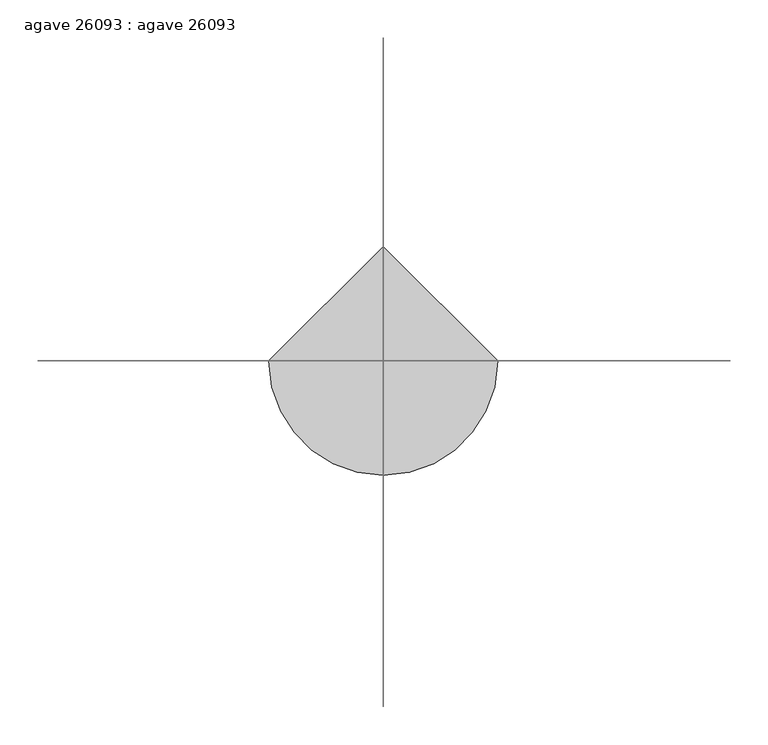
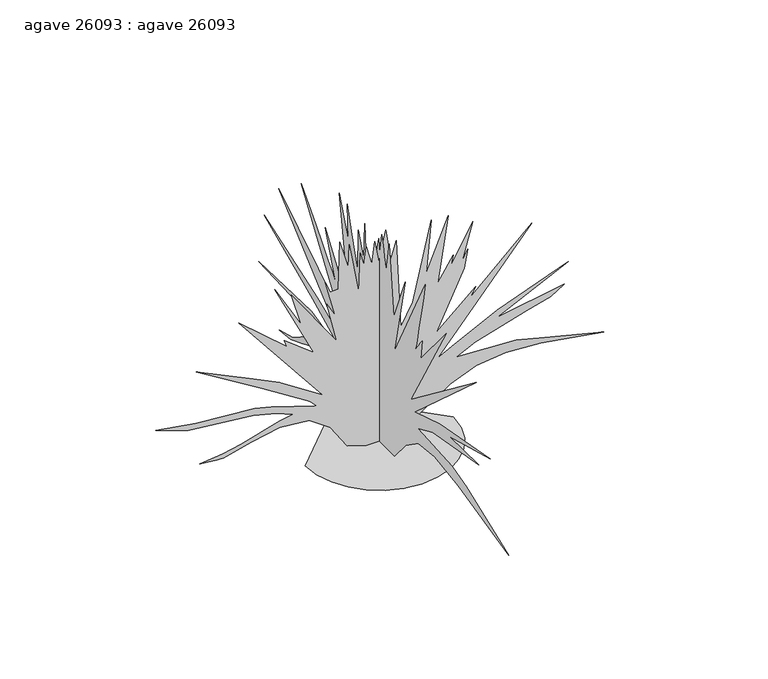
"""IFC4 building model written with IfcOpenShell, lengths in millimetres: proxy geometry, agave 26093 : agave 26093."""

from ifc_helpers import new_model, si_unit, origin, place, context, project, spatial, triangles, source, transform, mapped, element, save


def agave_26093_agave_26093_93a2a214(model_context):
    return source(origin(), model_context, "Body", "Tessellation", [
        triangles([(-150.7087333, 0.0, 9.4e-06), (-146.7244834, -34.5323444, 9.4e-06), (-135.3772836, -66.2450299, 9.4e-06), (-117.5759356, -94.2289958, 9.4e-06), (-94.2289958, -117.5759356, 9.4e-06), (-66.2450299, -135.3772836, 9.4e-06), (-34.5323444, -146.7244834, 9.4e-06), (6.6e-06, -150.7087333, 9.4e-06), (34.5323444, -146.7244834, 9.4e-06), (66.2450299, -135.3772836, 9.4e-06), (94.2289958, -117.5759356, 9.4e-06), (117.5759356, -94.2289958, 9.4e-06), (135.3772836, -66.2450299, 9.4e-06), (146.7244834, -34.5323444, 9.4e-06), (150.7087333, 1.32e-05, 9.4e-06), (-1.98e-05, 150.7087333, 9.4e-06), (-24.9398476, 1.1e-06, 2.5e-06), (-65.4258802, 2.1e-06, 13.141818), (-99.6620581, 5e-07, 65.0964399), (-143.0435126, 6e-07, 95.6658721), (-202.3246234, 2.8e-06, 101.1403381), (-259.7355268, 6e-06, 89.1792132), (-316.7763402, 9.4e-06, 74.9889865), (-329.6211594, 9.9e-06, 75.5035945), (-365.3285002, 1.12e-05, 79.1975187), (-318.313056, 8.9e-06, 84.1103911), (-282.3389982, 6.9e-06, 91.7898278), (-203.1008479, 2e-06, 114.8573697), (-175.7107319, 5e-07, 119.829677), (-208.3624635, 1.2e-06, 133.0887423), (-256.7688111, 2.5e-06, 145.787731), (-389.2832517, 7.5e-06, 160.0767662), (-455.2115313, 9e-06, 182.6248811), (-373.9467241, 6.3e-06, 169.0808314), (-253.2813787, 1.6e-06, 159.2306877), (-220.3573709, 6e-07, 151.0805947), (-127.6907252, -1.6e-06, 121.0610699), (-140.4735387, -1.9e-06, 135.3043865), (-238.3492232, -1.3e-06, 197.06021), (-372.7148226, -4e-07, 279.8955245), (-256.342093, -2.1e-06, 224.048243), (-204.0302424, -2.9e-06, 198.6317166), (-115.3780683, -3.3e-06, 140.7615752), (-286.5249345, -8.6e-06, 355.0033673), (-188.0233888, -7.9e-06, 270.045399), (-192.9487059, -8.5e-06, 284.8205873), (-133.8471808, -8.3e-06, 238.0324729), (-212.6492294, -1.47e-05, 401.7927715), (-158.472758, -1.14e-05, 306.9846414), (-179.4046562, -1.47e-05, 378.3993593), (-87.0585669, -1.09e-05, 246.6514781), (-106.7590813, -1.52e-05, 332.8418567), (-89.5210982, -1.41e-05, 302.0595786), (-110.4530055, -1.79e-05, 380.860619), (-99.717687, -1.69e-05, 356.9287222), (-83.2732056, -1.76e-05, 356.9490335), (-80.9021112, -2.37e-05, 457.2003633), (-63.426897, -2.09e-05, 396.9718449), (-61.2016014, -2.38e-05, 444.8864347), (-41.5013458, -1.82e-05, 335.3031163), (-39.0385601, -2.33e-05, 419.0317629), (-31.650966, -2.19e-05, 390.7107445), (-26.7259009, -2.44e-05, 428.8818884), (-15.6443803, -2.24e-05, 387.0175833), (-9.4879996, -2.54e-05, 433.8069511), (-0.8690236, -2.3e-05, 387.0175833), (12.6750416, -2.74e-05, 451.043399), (23.7565623, -2.39e-05, 383.3244221), (34.8381601, -2.66e-05, 420.261121), (43.4571494, -1.56e-05, 230.6448788), (68.0824677, -1.94e-05, 276.2023633), (105.4982208, -3.08e-05, 439.9537416), (95.1708261, -2.38e-05, 329.146152), (140.4829403, -3.22e-05, 436.9539974), (118.5650104, -2.3e-05, 299.5957755), (150.578436, -2.74e-05, 348.8489465), (145.6533642, -2.58e-05, 326.6848924), (189.9794467, -3.25e-05, 406.7178343), (167.81641, -2.69e-05, 327.9167939), (180.1290669, -2.88e-05, 351.3102061), (173.4681726, -2.62e-05, 313.009528), (116.102479, -1.66e-05, 193.7063995), (196.1359024, -2.44e-05, 265.1203362), (183.8229911, -2.26e-05, 244.1889286), (310.6447741, -3.51e-05, 361.1603316), (118.5650104, -1.34e-05, 138.2987895), (158.4747927, -1.63e-05, 158.0775423), (240.4617396, -2.24e-05, 198.6317166), (384.5207517, -3.19e-05, 252.8079337), (239.2306011, -2.13e-05, 182.6248811), (376.7864491, -2.88e-05, 206.3655105), (349.174072, -2.66e-05, 189.8819236), (300.4111145, -2.36e-05, 176.0696308), (195.4584909, -1.73e-05, 146.0828801), (156.7348917, -1.44e-05, 127.2172711), (278.6305944, -1.94e-05, 121.0610699), (336.3953462, -2.1e-05, 106.1004551), (457.1673348, -2.45e-05, 75.5035945), (329.0750444, -2.01e-05, 96.2046111), (257.431743, -1.73e-05, 101.1027496), (197.4574787, -1.42e-05, 94.105802), (144.7537007, -1.07e-05, 73.3684686), (86.5066293, -5.8e-06, 34.1325482), (33.0588878, -1.4e-06, 0.0), (9e-07, 20.0836192, 9.1e-06), (2.1e-06, 47.8000438, 9.9e-06), (3.7e-06, 68.4088604, 20.0829062), (6.2e-06, 99.6950775, 59.1195655), (8.3e-06, 132.7178983, 80.7177112), (1.03e-05, 174.2748821, 84.8467378), (1.15e-05, 208.5839434, 72.8693576), (1.35e-05, 272.2425033, 45.8366235), (1.48e-05, 311.9833551, 30.2844433), (1.65e-05, 353.3269798, 25.0212039), (1.48e-05, 305.3793614, 38.860505), (1.34e-05, 249.7515432, 74.8251566), (1.18e-05, 199.8564965, 97.660536), (1.01e-05, 161.2479701, 96.4354927), (1.17e-05, 188.527337, 110.366392), (1.51e-05, 256.1160167, 122.0234748), (2.29e-05, 425.717038, 129.5510222), (1.47e-05, 238.8183625, 134.6051196), (1.09e-05, 164.9452008, 118.743824), (8.2e-06, 119.3844099, 96.4354927), (1.1e-05, 159.9457058, 127.6671074), (1.54e-05, 233.8196305, 165.2718342), (2.53e-05, 406.273312, 240.4952587), (1.5e-05, 217.8867004, 177.6998184), (1.1e-05, 147.7036569, 148.1491784), (2.57e-05, 354.5588814, 329.146152), (1.25e-05, 146.2032761, 198.5547591), (2.38e-05, 274.5259576, 388.2494848), (2.18e-05, 248.7817623, 359.4966614), (1.99e-05, 223.9913424, 331.6328098), (1.81e-05, 201.1074557, 305.5495545), (1.65e-05, 181.0833509, 282.1358129), (1.52e-05, 164.872549, 262.2780679), (1.42e-05, 153.4283166, 246.8711776), (1.37e-05, 147.7036569, 236.8013344), (1.88e-05, 190.798601, 345.1532418), (1.51e-05, 148.9134577, 283.7461616), (1.48e-05, 144.9251474, 278.3410409), (1.44e-05, 140.1001603, 272.7403471), (1.4e-05, 134.5776867, 266.9770725), (1.35e-05, 128.4971803, 261.086807), (1.31e-05, 121.9980766, 255.0974924), (1.26e-05, 115.2200837, 249.0439011), (1.21e-05, 108.3028915, 242.95779), (1.97e-05, 140.3160628, 449.8114975), (1.58e-05, 109.53403, 367.3172959), (1.82e-05, 113.2279542, 442.4251751), (1.61e-05, 98.452766, 393.1745476), (1.29e-05, 75.0583319, 320.5279281), (1.55e-05, 73.826939, 410.4109955), (1.32e-05, 55.357822, 358.699072), (1.53e-05, 51.6638932, 437.5001123), (1.36e-05, 47.2595336, 384.1829453), (1.1e-05, 27.0383205, 327.9167939), (1.31e-05, 1.1814591, 436.2682108), (1.2e-05, -1.2811313, 405.4859327), (1.3e-05, -8.5500533, 450.4566616), (1.25e-05, -11.9783704, 436.1437634), (1.19e-05, -15.2441015, 422.2677209), (1.14e-05, -18.1847128, 409.2629188), (1.09e-05, -20.6375916, 397.5687561), (1.05e-05, -22.4401819, 387.6195451), (1.03e-05, -23.4298925, 379.852214), (1.01e-05, -23.4441676, 374.7036547), (1.18e-05, -34.5257405, 446.1183363), (6.6e-06, -50.5323262, 298.3664174), (7.8e-06, -92.3958773, 399.3315119), (4.4e-06, -52.9948575, 225.7198161), (5.7e-06, -162.5786665, 436.2682108), (5.1e-06, -155.9520543, 404.0000133), (4.4e-06, -149.5159464, 372.9078704), (3.8e-06, -143.4613468, 344.1651844), (3.3e-06, -137.9787509, 318.9480463), (2.9e-06, -133.2591716, 298.4324563), (2.7e-06, -129.4933677, 283.7918891), (2.6e-06, -126.87158, 276.2023633), (2.5e-06, -126.0089964, 274.2135312), (2.5e-06, -127.1682462, 275.2524031), (2.5e-06, -130.0120315, 278.8160301), (2.5e-06, -134.204054, 284.398956), (2.5e-06, -139.4067433, 291.4957067), (2.4e-06, -145.2835467, 299.6034059), (2.4e-06, -151.4971481, 308.2165429), (1.4e-06, -145.3409469, 266.3522378), (6e-07, -236.4556433, 375.9355562), (-2e-07, -110.8649898, 157.9992949), (-5.3e-06, -341.1146439, 334.0712148), (-1.4e-06, -124.4090487, 138.2990438), (-4.6e-06, -213.0612137, 166.6183), (-1.15e-05, -391.2898516, 199.4396978), (-6.2e-06, -246.3057688, 160.4618262), (-1.09e-05, -351.4651749, 162.9246119), (-4.5e-06, -189.3266705, 133.5012353), (-2.8e-06, -135.490567, 109.9795515), (-8.4e-06, -257.3885589, 102.5916939), (-1.11e-05, -306.6392046, 89.0476442), (-1.94e-05, -455.623025, 31.1775097), (-1.03e-05, -278.0057598, 72.8693576), (-6.2e-06, -195.1343828, 85.0082832), (-3.8e-06, -137.6096873, 78.9734862), (-2.8e-06, -94.1832773, 48.8668437), (-2.4e-06, -52.6021717, 6.9e-06), (-9e-07, -19.1255291, 7.9e-06)], [[15, 16, 1], [14, 15, 1], [14, 1, 2], [13, 14, 2], [13, 2, 3], [13, 3, 4], [12, 13, 4], [11, 12, 4], [11, 4, 5], [11, 5, 6], [11, 6, 7], [11, 7, 8], [11, 8, 9], [11, 9, 10], [47, 48, 49], [97, 98, 99], [88, 89, 90], [39, 40, 41], [84, 85, 86], [71, 72, 73], [53, 54, 55], [32, 33, 34], [43, 44, 45], [24, 25, 26], [58, 59, 60], [77, 78, 79], [73, 74, 75], [60, 61, 62], [51, 52, 53], [56, 57, 58], [82, 83, 84], [79, 80, 81], [64, 65, 66], [49, 50, 51], [68, 69, 70], [75, 76, 77], [90, 91, 92], [90, 92, 93], [66, 67, 68], [82, 84, 86], [90, 93, 94], [62, 63, 64], [47, 49, 51], [39, 41, 42], [45, 46, 47], [43, 45, 47], [38, 39, 42], [38, 42, 43], [31, 32, 34], [31, 34, 35], [23, 24, 26], [56, 58, 60], [87, 88, 90], [87, 90, 94], [87, 94, 95], [37, 38, 43], [86, 87, 95], [71, 73, 75], [96, 97, 99], [96, 99, 100], [95, 96, 100], [95, 100, 101], [95, 101, 102], [53, 55, 56], [53, 56, 60], [22, 23, 26], [22, 26, 27], [22, 27, 28], [21, 22, 28], [60, 62, 64], [43, 47, 51], [30, 31, 35], [30, 35, 36], [30, 36, 37], [29, 30, 37], [86, 95, 102], [21, 28, 29], [20, 21, 29], [20, 29, 37], [19, 20, 37], [86, 102, 103], [66, 68, 70], [64, 66, 70], [60, 64, 70], [53, 60, 70], [51, 53, 70], [43, 51, 70], [77, 79, 81], [77, 81, 82], [75, 77, 82], [71, 75, 82], [70, 71, 82], [70, 82, 86], [43, 70, 86], [43, 86, 103], [43, 103, 104], [43, 104, 17], [43, 17, 18], [43, 18, 19], [43, 19, 37], [120, 121, 122], [193, 194, 195], [190, 191, 192], [126, 127, 128], [155, 156, 157], [131, 132, 133], [200, 201, 202], [113, 114, 115], [195, 196, 197], [129, 130, 131], [131, 133, 134], [170, 171, 172], [188, 189, 190], [131, 134, 135], [148, 149, 150], [139, 140, 141], [131, 135, 136], [150, 151, 152], [168, 169, 170], [172, 173, 174], [131, 136, 137], [158, 159, 160], [172, 174, 175], [131, 137, 138], [153, 154, 155], [131, 138, 139], [172, 175, 176], [160, 161, 162], [172, 176, 177], [186, 187, 188], [172, 177, 178], [112, 113, 115], [112, 115, 116], [111, 112, 116], [111, 116, 117], [160, 162, 163], [172, 178, 179], [172, 179, 180], [172, 180, 181], [139, 141, 142], [193, 195, 197], [185, 186, 188], [192, 193, 197], [192, 197, 198], [155, 157, 158], [150, 152, 153], [148, 150, 153], [139, 142, 143], [199, 200, 202], [119, 120, 122], [119, 122, 123], [118, 119, 123], [199, 202, 203], [198, 199, 203], [198, 203, 204], [184, 185, 188], [110, 111, 117], [110, 117, 118], [109, 110, 118], [160, 163, 164], [118, 123, 124], [109, 118, 124], [139, 143, 144], [125, 126, 128], [125, 128, 129], [183, 184, 188], [139, 144, 145], [153, 155, 158], [108, 109, 124], [139, 145, 146], [160, 164, 165], [158, 160, 165], [158, 165, 166], [158, 166, 167], [158, 167, 168], [158, 168, 170], [182, 183, 188], [124, 125, 129], [182, 188, 190], [181, 182, 190], [172, 181, 190], [139, 146, 147], [131, 139, 147], [131, 147, 148], [158, 170, 172], [153, 158, 172], [148, 153, 172], [198, 204, 205], [131, 148, 172], [129, 131, 172], [124, 129, 172], [124, 172, 190], [108, 124, 190], [107, 108, 190], [106, 107, 190], [105, 106, 190], [207, 105, 190], [206, 207, 190], [205, 206, 190], [198, 205, 190], [192, 198, 190]], closed=False),
    ])


if __name__ == "__main__":
    model = new_model("IFC4")
    model_context = context("Model", 3, world=origin())
    ifc_project = project(units=[si_unit("LENGTHUNIT", "METRE", prefix="MILLI")], contexts=[model_context])
    site = spatial("IfcSite", under=ifc_project)
    building = spatial("IfcBuilding", under=site)
    placement = place(None, origin())
    agave_26093_agave_26093_shape = agave_26093_agave_26093_93a2a214(model_context)
    element("IfcBuildingElementProxy", 1, Name="agave 26093 : agave 26093", ObjectType="agave 26093 : agave 26093", at=placement, inside=building, context=model_context, shape_type="MappedRepresentation", body=[
        mapped(agave_26093_agave_26093_shape, transform((0.0, 0.0, 0.0), x_axis=(1.0, 0.0, 0.0), y_axis=(0.0, 1.0, 0.0), z_axis=(0.0, 0.0, 1.0))),
    ])
    save(model, "model.ifc")

# Revit data of these elements
# Type "agave 26093 : agave 26093"
#   built-in parameter 1005195 = "RPC-16-G1GJ-63FX-7K5P-N000-ST1L-LVER-AU"
#   Height = 0
